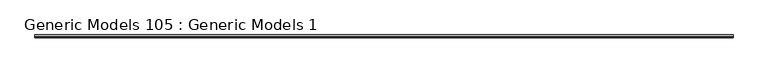
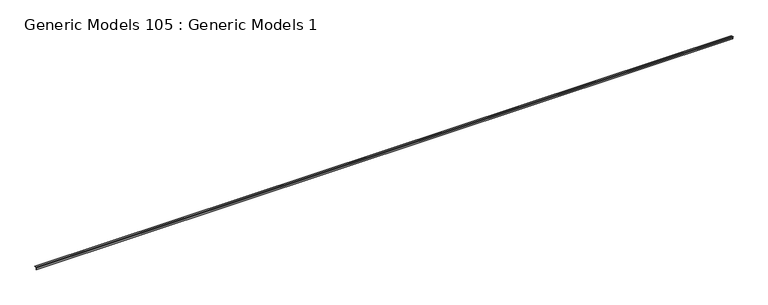
"""IFC4 building model written with IfcOpenShell, lengths in millimetres: proxy geometry, Generic Models 105 : Generic Models 1."""

from ifc_helpers import new_model, si_unit, point, frame, frame_2d, origin, place, context, project, spatial, polyline, circle_curve, trimmed, segment, composite_curve, outline, extrude, source, transform, mapped, element, save


def generic_models_105_generic_models_1_ee0505f5(model_context):
    return source(origin(), model_context, "Body", "SweptSolid", [
        extrude(outline(composite_curve([segment(polyline([(51259.8971572, 127166.5926156), (51297.9226718, 127147.066), (51336.0226718, 127147.066), (51336.0226718, 127145.796), (51297.6156481, 127145.796), (51258.8625498, 127165.6962396), (51278.7627895, 127126.9431414), (51278.7627895, 127088.5361176), (51277.4927895, 127088.5361176), (51277.4927895, 127126.6361176), (51257.9661739, 127164.6616323)]), True, "CONTINUOUS"), segment(trimmed(circle_curve(frame_2d((51259.2420022, 127165.3167873)), 1.4342127), [point((51257.9661739, 127164.6616323))], [point((51259.8971572, 127166.5926156))], False, "CARTESIAN"), True, "CONTINUOUS")], self_intersect=False)), frame((-20998.9733045, 0.0, 0.0), z_axis=(1.0, 0.0, 0.0), x_axis=(0.0, 1.0, 0.0)), (0.0, 0.0, 1.0), 19050.0),
    ])


if __name__ == "__main__":
    model = new_model("IFC4")
    model_context = context("Model", 3, world=origin())
    ifc_project = project(units=[si_unit("LENGTHUNIT", "METRE", prefix="MILLI")], contexts=[model_context])
    site = spatial("IfcSite", under=ifc_project)
    building = spatial("IfcBuilding", under=site)
    placement = place(None, origin())
    generic_models_105_generic_models_1_shape = generic_models_105_generic_models_1_ee0505f5(model_context)
    element("IfcBuildingElementProxy", 1, Name="Generic Models 105 : Generic Models 1", ObjectType="Generic Models 105 : Generic Models 1", at=placement, inside=building, context=model_context, shape_type="MappedRepresentation", body=[
        mapped(generic_models_105_generic_models_1_shape, transform((0.0, 0.0, 0.0), x_axis=(1.0, 0.0, 0.0), y_axis=(0.0, 1.0, 0.0), z_axis=(0.0, 0.0, 1.0))),
    ])
    save(model, "model.ifc")

# Revit data of these elements
# Element 1 (IfcBuildingElementProxy, "Generic Models 105 : Generic Models 1")
#   Materials on its faces: "_CONTINIOUS 16 GA. COPPER CORNER BEAD"
# Materials
#   "_CONTINIOUS 16 GA. COPPER CORNER BEAD": class "Generic", colour RGB 253 192 103, transparency 0, Cost = 0
